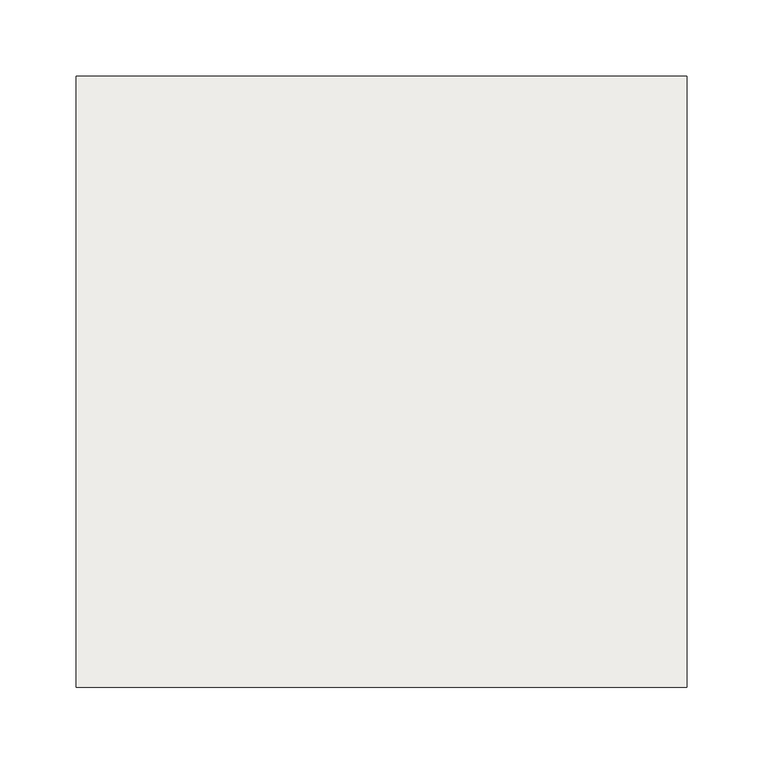
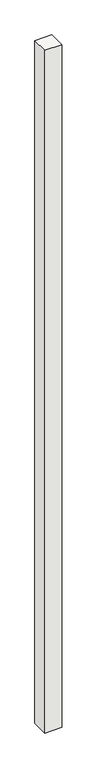
"""IFC4 building model written with IfcOpenShell, lengths in millimetres: footing geometry, NLRS_17_SFO_TLB_funderingspaal geheid beton prefab-AV-MMBPC_gen_rsf : heipaal beton prefab_gen__bxh 400x400."""

from ifc_helpers import new_model, si_unit, frame, origin, place, context, project, spatial, polyline, outline, extrude, source, transform, mapped, element, save


def footing_f9187350(model_context):
    return source(origin(), model_context, "Body", "SweptSolid", [
        extrude(outline(polyline([(200.0, -200.0), (-200.0, -200.0), (-200.0, 200.0), (200.0, 200.0), (200.0, -200.0)])), frame((0.0, 0.0, -20000.0), z_axis=(0.0, 0.0, 1.0), x_axis=(1.0, 0.0, 0.0)), (0.0, 0.0, 1.0), 16925.0),
    ])


if __name__ == "__main__":
    model = new_model("IFC4")
    model_context = context("Model", 3, world=origin())
    ifc_project = project(units=[si_unit("LENGTHUNIT", "METRE", prefix="MILLI")], contexts=[model_context])
    site = spatial("IfcSite", under=ifc_project)
    building = spatial("IfcBuilding", under=site)
    placement = place(None, origin())
    footing_shape = footing_f9187350(model_context)
    element("IfcFooting", 1, ObjectType="NLRS_17_SFO_TLB_funderingspaal geheid beton prefab-AV-MMBPC_gen_rsf : heipaal beton prefab_gen__bxh 400x400", at=placement, inside=building, context=model_context, shape_type="MappedRepresentation", body=[
        mapped(footing_shape, transform((0.0, 0.0, 0.0), x_axis=(1.0, 0.0, 0.0), y_axis=(0.0, 1.0, 0.0), z_axis=(0.0, 0.0, 1.0))),
    ])
    save(model, "model.ifc")

# Revit data of these elements
# Type "NLRS_17_SFO_TLB_funderingspaal geheid beton prefab-AV-MMBPC_gen_rsf : heipaal beton prefab_gen__bxh 400x400"
#   IfcExportAs = "IfcPile"
#   Type Comments = "prefab heipaal 400x400"
#   Model = " "
#   Manufacturer = " "
#   Description = "prefab heipaal 400x400"
#   Assembly Code = "17.21"
#   Width = 400 mm
#   Slanted Angle [instance default] = 0.00°
#   NLRS_S_draagvermogen_trek [instance default] = 0.00 kN
#   NLRS_S_draagvermogen_druk [instance default] = 0.00 kN
#   NLRS_C_lengte [instance default] = 1660 mm
#   NLRS_C_hoogte = 400 mm
#   NLRS_C_breedte = 400 mm
#   Height [instance default] = 1660 mm
#   Length [instance default] = 1660 mm
#   Angle [instance default] = 0.00°
#   Slanted [instance default] = 0
#   Structural Material = NLRS_f2_beton prefab_gen_rsf
#   Keynote = ""
# Element 1 (IfcFooting, "NLRS_17_SFO_TLB_funderingspaal geheid beton prefab-AV-MMBPC_gen_rsf : heipaal beton prefab_gen__bxh 400x400")
#   NLRS_C_lengte = 16925 mm
#   Height = 16925 mm
#   Length = 16925 mm
#   Materials on its faces: "NLRS_f2_beton prefab_gen_rsf"
# Materials
#   "NLRS_f2_beton prefab_gen_rsf": class "F - Niet gebakken kunststeen", colour RGB 129 133 118, transparency 0, Keynote = "f2", Manufacturer = "Revit Standards Foundation", URL = "www.revitstandards.org", Description = "beton prefab", Cost = 0
